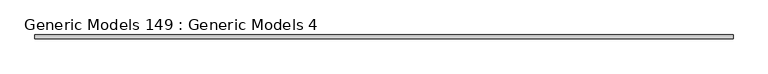
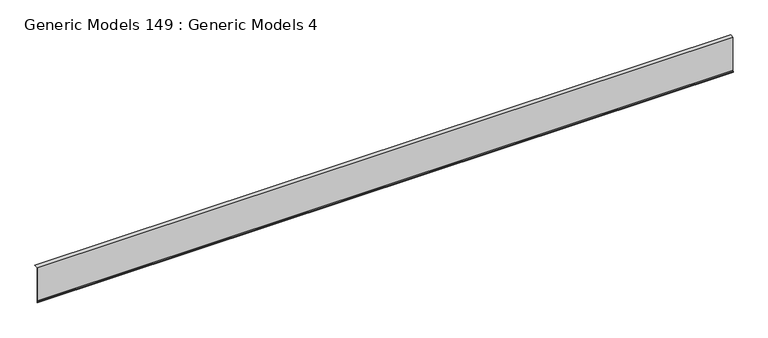
"""IFC4 building model written with IfcOpenShell, lengths in millimetres: proxy geometry, Generic Models 149 : Generic Models 4."""

import ifcopenshell
import ifcopenshell.guid

model = None  # the IFC model being written
_history = None  # IfcOwnerHistory: only IFC2X3 demands one
_inside = {}  # id of a spatial element -> (the spatial element, [elements in it])
_under = {}  # id of a project, library or spatial element -> (it, [spatial elements below it])
_declared = {}  # id of a project -> (the project, [libraries it declares])
_typed = {}  # id of a type object -> (the type object, [elements of that type])
_made_of = {}  # id of a material, layer set ... -> (it, [elements and type objects made of it])


def new_model(schema):
    """Start an empty IFC model of exactly this schema.

    Asked for "IFC4X3", IfcOpenShell would pick the latest addendum, in which some entities
    have other attributes; the version numbers below select the first issue.
    IFC2X3 requires an IfcOwnerHistory on every rooted entity: one is made here for all.
    """
    global model, _history
    if schema == "IFC4X3":
        model = ifcopenshell.file(schema_version=(4, 3, 0, 0))
    else:
        model = ifcopenshell.file(schema=schema)
    _inside.clear()
    _under.clear()
    _declared.clear()
    _typed.clear()
    _made_of.clear()
    _history = None
    if model.schema == "IFC2X3":
        org = make("IfcOrganization", Name="unknown")
        user = make(
            "IfcPersonAndOrganization",
            ThePerson=make("IfcPerson", FamilyName="unknown"),
            TheOrganization=org,
        )
        app = make(
            "IfcApplication",
            ApplicationDeveloper=org,
            Version="unknown",
            ApplicationFullName="unknown",
            ApplicationIdentifier="unknown",
        )
        _history = make(
            "IfcOwnerHistory",
            OwningUser=user,
            OwningApplication=app,
            ChangeAction="ADDED",
            CreationDate=0,
        )
    return model


def make(cls, **values):
    """One entity of the class cls with the attributes given. An attribute that is None is left unset."""
    return model.create_entity(
        cls, **{name: value for name, value in values.items() if value is not None}
    )


def rooted(cls, **values):
    """An entity with a GlobalId (a new one), such as an element, a storey or a relation."""
    return make(cls, GlobalId=ifcopenshell.guid.new(), OwnerHistory=_history, **values)


def si_unit(unit_type, name, prefix=None):
    """IfcSIUnit, for example si_unit("LENGTHUNIT", "METRE", prefix="MILLI")."""
    return make("IfcSIUnit", UnitType=unit_type, Prefix=prefix, Name=name)


def assignment(units):
    """IfcUnitAssignment: the units of a project."""
    return None if units is None else make("IfcUnitAssignment", Units=units)


def point(xyz):
    """IfcCartesianPoint."""
    return None if xyz is None else make("IfcCartesianPoint", Coordinates=xyz)


def direction(xyz):
    """IfcDirection."""
    return None if xyz is None else make("IfcDirection", DirectionRatios=xyz)


def frame(location, z_axis=None, x_axis=None):
    """IfcAxis2Placement3D, a coordinate frame: its origin and axes. An axis left out is left unset."""
    return make(
        "IfcAxis2Placement3D",
        Location=point(location),
        Axis=direction(z_axis),
        RefDirection=direction(x_axis),
    )


def origin():
    """The frame at (0, 0, 0) with its axes left unset."""
    return frame((0.0, 0.0, 0.0))


def place(relative_to, where):
    """IfcLocalPlacement: puts the frame where relative to a parent placement (None: the world)."""
    return make(
        "IfcLocalPlacement", PlacementRelTo=relative_to, RelativePlacement=where
    )


def context(
    kind, dimensions, precision=None, world=None, true_north=None, identifier=None
):
    """IfcGeometricRepresentationContext, for example the 3D "Model" context."""
    return make(
        "IfcGeometricRepresentationContext",
        ContextIdentifier=identifier,
        ContextType=kind,
        CoordinateSpaceDimension=dimensions,
        Precision=precision,
        WorldCoordinateSystem=world,
        TrueNorth=true_north,
    )


def project(units=None, contexts=None):
    """IfcProject with its units and contexts."""
    return rooted(
        "IfcProject",
        Name="project",
        RepresentationContexts=contexts,
        UnitsInContext=assignment(units),
    )


def spatial(cls, under=None, at=None, **own):
    """A site, building, storey or space (cls), placed at a placement, below another one or the project."""
    s = rooted(cls, ObjectPlacement=at, **own)
    if under is not None:
        _under.setdefault(under.id(), (under, []))[1].append(s)
    return s


def polyline(points):
    """IfcPolyline through the points."""
    return make("IfcPolyline", Points=[point(p) for p in points])


def outline(outer, holes=None, kind="AREA"):
    """IfcArbitraryClosedProfileDef: a profile drawn as a closed curve; with holes, ...WithVoids."""
    if holes is None:
        return make("IfcArbitraryClosedProfileDef", ProfileType=kind, OuterCurve=outer)
    return make(
        "IfcArbitraryProfileDefWithVoids",
        ProfileType=kind,
        OuterCurve=outer,
        InnerCurves=holes,
    )


def extrude(swept, where, along, depth):
    """IfcExtrudedAreaSolid: the profile swept, set in the frame where, extruded along a direction by depth."""
    return make(
        "IfcExtrudedAreaSolid",
        SweptArea=swept,
        Position=where,
        ExtrudedDirection=direction(along),
        Depth=depth,
    )


def shape(context_of_items, identifier, shape_type, items):
    """IfcShapeRepresentation: the items that make up one representation, for example the "Body"."""
    return make(
        "IfcShapeRepresentation",
        ContextOfItems=context_of_items,
        RepresentationIdentifier=identifier,
        RepresentationType=shape_type,
        Items=items,
    )


def source(mapping_origin, context_of_items, identifier, shape_type, items):
    """IfcRepresentationMap: a shape defined once, which mapped items show again and again."""
    return make(
        "IfcRepresentationMap",
        MappingOrigin=mapping_origin,
        MappedRepresentation=shape(context_of_items, identifier, shape_type, items),
    )


def transform(
    local_origin,
    x_axis=None,
    y_axis=None,
    z_axis=None,
    scale=None,
    scale2=None,
    scale3=None,
    uniform=True,
):
    """IfcCartesianTransformationOperator3D, or its non-uniform kind. x_axis, y_axis, z_axis: its Axis1, 2, 3."""
    if uniform:
        return make(
            "IfcCartesianTransformationOperator3D",
            Axis1=direction(x_axis),
            Axis2=direction(y_axis),
            LocalOrigin=point(local_origin),
            Scale=scale,
            Axis3=direction(z_axis),
        )
    return make(
        "IfcCartesianTransformationOperator3DnonUniform",
        Axis1=direction(x_axis),
        Axis2=direction(y_axis),
        LocalOrigin=point(local_origin),
        Scale=scale,
        Axis3=direction(z_axis),
        Scale2=scale2,
        Scale3=scale3,
    )


def mapped(mapping_source, mapping_target):
    """IfcMappedItem: shows the shape of a source again, moved by a transform."""
    return make(
        "IfcMappedItem", MappingSource=mapping_source, MappingTarget=mapping_target
    )


def made_of(thing, what):
    """Note that an element or type object is made of a material, layer set ...; save() writes the relation."""
    if what is not None:
        _made_of.setdefault(what.id(), (what, []))[1].append(thing)
    return thing


def element(
    cls,
    number,
    at=None,
    inside=None,
    cuts=None,
    type_object=None,
    material=None,
    context=None,
    identifier="Body",
    shape_type=None,
    held_by="IfcProductDefinitionShape",
    body=None,
    shapes=None,
    **own,
):
    """One element of the class cls, such as IfcWall. Its Tag is "e" and its number.

    at: its placement. inside: the storey or other place that contains it. cuts: it is an
    opening in that element (IfcRelVoidsElement). A single representation is given by context,
    identifier, shape_type and body (its items); several are given by shapes. held_by: the class
    of the entity that holds the representations. save() writes the other relations.
    """
    e = rooted(cls, Tag="e%d" % number, ObjectPlacement=at, **own)
    if body is not None:
        shapes = [shape(context, identifier, shape_type, body)]
    if shapes is not None:
        e.Representation = make(held_by, Representations=shapes)
    if inside is not None:
        _inside.setdefault(inside.id(), (inside, []))[1].append(e)
    if cuts is not None:
        rooted(
            "IfcRelVoidsElement", RelatingBuildingElement=cuts, RelatedOpeningElement=e
        )
    if type_object is not None:
        _typed.setdefault(type_object.id(), (type_object, []))[1].append(e)
    return made_of(e, material)


def aggregate(whole, parts):
    """IfcRelAggregates: a whole, such as a stair, and the parts it consists of."""
    return rooted("IfcRelAggregates", RelatingObject=whole, RelatedObjects=parts)


def save(model, path):
    """Write the relations noted so far, then the file.

    IfcRelAggregates (storeys below a building ...), IfcRelContainedInSpatialStructure (elements
    in a storey), IfcRelDefinesByType, IfcRelAssociatesMaterial and IfcRelDeclares: one each for
    every whole, place, type object, material and project.
    """
    for whole, parts in _under.values():
        aggregate(whole, parts)
    for where, things in _inside.values():
        rooted(
            "IfcRelContainedInSpatialStructure",
            RelatedElements=things,
            RelatingStructure=where,
        )
    for kind, things in _typed.values():
        rooted("IfcRelDefinesByType", RelatedObjects=things, RelatingType=kind)
    for what, things in _made_of.values():
        rooted("IfcRelAssociatesMaterial", RelatedObjects=things, RelatingMaterial=what)
    for by, libraries in _declared.values():
        rooted("IfcRelDeclares", RelatingContext=by, RelatedDefinitions=libraries)
    model.write(path)


def generic_models_149_generic_models_4_ca827802(model_context):
    return source(origin(), model_context, "Body", "SweptSolid", [
        extrude(outline(polyline([(6876.7283206, 124206.052611), (6876.7283206, 123261.0407867), (6871.4999022, 123246.6758251), (6871.4999022, 123210.2265476), (6870.7061522, 123210.2265476), (6870.7061522, 123246.8157847), (6875.9345706, 123261.1807462), (6875.9345706, 124206.846361), (6976.0925912, 124206.846361), (6976.0925912, 124206.052611), (6876.7283206, 124206.052611)])), frame((-10234.5171316, 0.0, 0.0), z_axis=(1.0, 0.0, 0.0), x_axis=(0.0, 1.0, 0.0)), (0.0, 0.0, 1.0), 18643.6),
    ])


if __name__ == "__main__":
    model = new_model("IFC4")
    model_context = context("Model", 3, world=origin())
    ifc_project = project(units=[si_unit("LENGTHUNIT", "METRE", prefix="MILLI")], contexts=[model_context])
    site = spatial("IfcSite", under=ifc_project)
    building = spatial("IfcBuilding", under=site)
    placement = place(None, origin())
    generic_models_149_generic_models_4_shape = generic_models_149_generic_models_4_ca827802(model_context)
    element("IfcBuildingElementProxy", 1, Name="Generic Models 149 : Generic Models 4", ObjectType="Generic Models 149 : Generic Models 4", at=placement, inside=building, context=model_context, shape_type="MappedRepresentation", body=[
        mapped(generic_models_149_generic_models_4_shape, transform((0.0, 0.0, 0.0), x_axis=(1.0, 0.0, 0.0), y_axis=(0.0, 1.0, 0.0), z_axis=(0.0, 0.0, 1.0))),
    ])
    save(model, "model.ifc")

# Revit data of these elements
# Element 1 (IfcBuildingElementProxy, "Generic Models 149 : Generic Models 4")
#   Materials on its faces: "_(2) LAYERS NO. 30 ASTM D226 ASPHALT SATURATED ORGANIC FELT"
# Materials
#   "_(2) LAYERS NO. 30 ASTM D226 ASPHALT SATURATED ORGANIC FELT": class "Generic", colour RGB 67 154 161, transparency 0, Cost = 0
